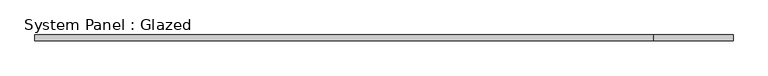
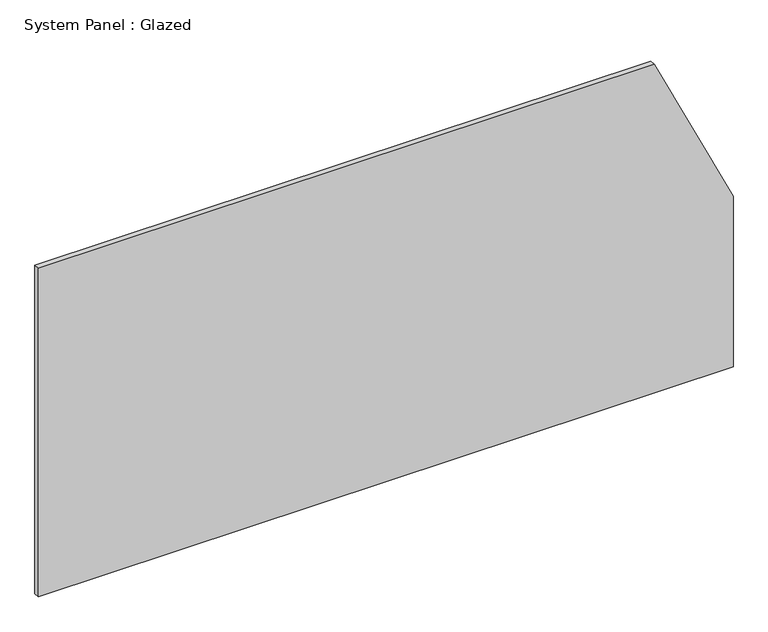
"""IFC4 building model written with IfcOpenShell, lengths in millimetres: plate geometry, System Panel : Glazed."""

from ifc_helpers import new_model, si_unit, frame, origin, place, context, project, spatial, polyline, outline, extrude, source, transform, mapped, element, save


def system_panel_glazed_93e257c1(model_context):
    return source(origin(), model_context, "Body", "SweptSolid", [
        extrude(outline(polyline([(0.0, -1500.0), (0.0, 1500.0), (779.2966956, 1500.0), (1500.0, 1159.42413), (1500.0, -1500.0), (0.0, -1500.0)])), frame((0.0, 24.5, 0.0), z_axis=(0.0, 1.0, 0.0), x_axis=(0.0, 0.0, 1.0)), (0.0, 0.0, 1.0), 25.0),
    ])


if __name__ == "__main__":
    model = new_model("IFC4")
    model_context = context("Model", 3, world=origin())
    ifc_project = project(units=[si_unit("LENGTHUNIT", "METRE", prefix="MILLI")], contexts=[model_context])
    site = spatial("IfcSite", under=ifc_project)
    building = spatial("IfcBuilding", under=site)
    placement = place(None, origin())
    system_panel_glazed_shape = system_panel_glazed_93e257c1(model_context)
    element("IfcPlate", 1, ObjectType="System Panel : Glazed", at=placement, inside=building, context=model_context, shape_type="MappedRepresentation", body=[
        mapped(system_panel_glazed_shape, transform((0.0, 0.0, 0.0), x_axis=(1.0, 0.0, 0.0), y_axis=(0.0, 1.0, 0.0), z_axis=(0.0, 0.0, 1.0))),
    ])
    save(model, "model.ifc")

# Revit data of these elements
# Type "System Panel : Glazed"
#   Construction Type Id = "GSP4R"
#   Analytic Construction = "1/8 in Pilkington single glazing"
#   Visual Light Transmittance = 0.9
#   Solar Heat Gain Coefficient = 0.86
#   Heat Transfer Coefficient (U) = 6.7069 W/(m²·K)
#   Define Thermal Properties by = 1
# Element 1 (IfcPlate, "System Panel : Glazed")
#   Materials on its faces: "Glass"
# Materials
#   "Glass": class "Glass", colour RGB 0 128 192, transparency 0.9, Description = "Soda Lime Glass", Cost = 0
